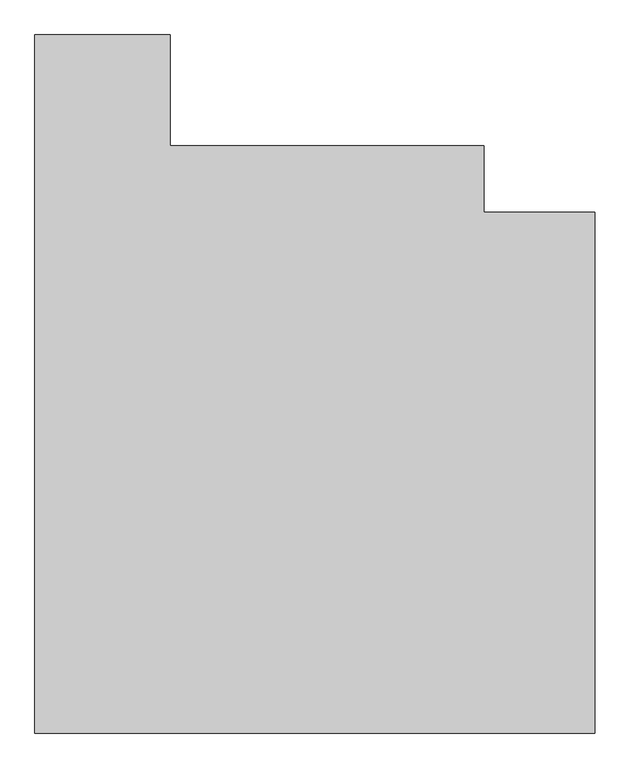
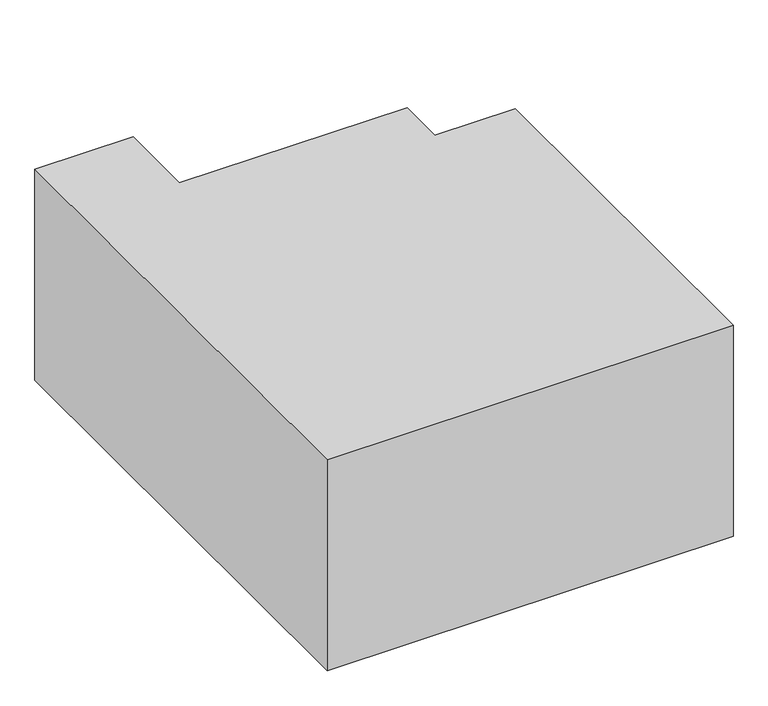
"""IFC4 building model written with IfcOpenShell, lengths in millimetres: proxy geometry, 0_3d_modell."""

from ifc_helpers import new_model, si_unit, origin, origin_with_axes, place, context, project, spatial, polyline, outline, extrude, source, transform, mapped, element, save


def generic_models_a6dc762b(model_context):
    return source(origin(), model_context, "Body", "SweptSolid", [
        extrude(outline(polyline([(0.0, 5670.0), (1100.0, 5670.0), (1100.0, 4770.0), (3650.0, 4770.0), (3650.0, 4230.0), (4550.0, 4230.0), (4550.0, 0.0), (0.0, 0.0), (0.0, 5670.0)])), origin_with_axes(), (0.0, 0.0, 1.0), 2500.0),
    ])


if __name__ == "__main__":
    model = new_model("IFC4")
    model_context = context("Model", 3, world=origin())
    ifc_project = project(units=[si_unit("LENGTHUNIT", "METRE", prefix="MILLI")], contexts=[model_context])
    site = spatial("IfcSite", under=ifc_project)
    building = spatial("IfcBuilding", under=site)
    placement = place(None, origin())
    generic_models_shape = generic_models_a6dc762b(model_context)
    element("IfcBuildingElementProxy", 1, Name="0_3d_modell", ObjectType="0_3d_modell", at=placement, inside=building, context=model_context, shape_type="MappedRepresentation", body=[
        mapped(generic_models_shape, transform((0.0, 0.0, 0.0), x_axis=(1.0, 0.0, 0.0), y_axis=(0.0, 1.0, 0.0), z_axis=(0.0, 0.0, 1.0))),
    ])
    save(model, "model.ifc")

# Revit data of these elements
# Element 1 (IfcBuildingElementProxy, "0_3d_modell")
#   Materials on its faces: "*1"
# Materials
#   "*1": class "Unassigned", colour RGB 175 175 175, transparency 0
